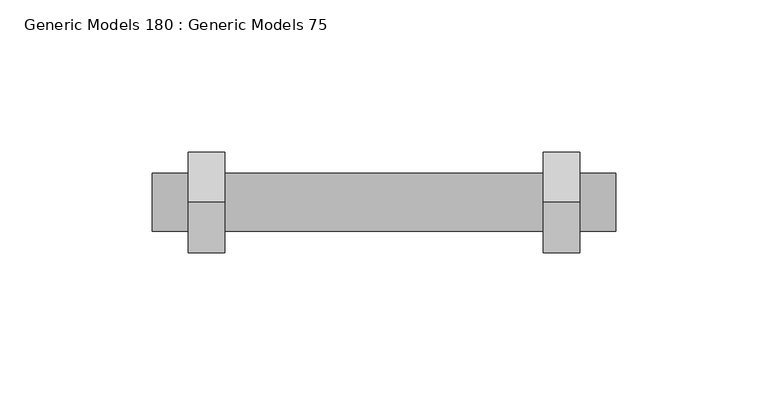
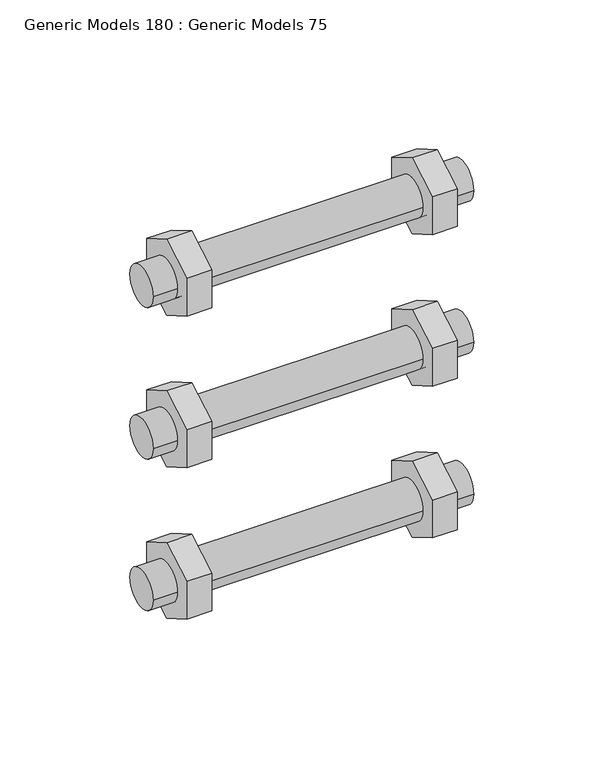
"""IFC4 building model written with IfcOpenShell, lengths in millimetres: proxy geometry, Generic Models 180 : Generic Models 75."""

from ifc_helpers import new_model, si_unit, point, frame, frame_2d, origin, place, context, project, spatial, polyline, circle_curve, trimmed, segment, composite_curve, outline, extrude, source, transform, mapped, element, save


def generic_models_180_generic_models_75_568aabff(model_context):
    return source(origin(), model_context, "Body", "SweptSolid", [
        extrude(outline(polyline([(30912.6241273, 269062.859622), (30929.1219112, 269072.384622), (30945.6196951, 269062.859622), (30945.6196951, 269043.809622), (30929.1219112, 269034.284622), (30912.6241273, 269043.809622), (30912.6241273, 269062.859622)])), frame((31918.2596032, 0.0, 0.0), z_axis=(1.0, 0.0, 0.0), x_axis=(0.0, 1.0, 0.0)), (0.0, 0.0, 1.0), 11.90625),
        extrude(outline(polyline([(30912.6241273, 268986.659622), (30929.1219112, 268996.184622), (30945.6196951, 268986.659622), (30945.6196951, 268967.609622), (30929.1219112, 268958.084622), (30912.6241273, 268967.609622), (30912.6241273, 268986.659622)])), frame((31918.2596032, 0.0, 0.0), z_axis=(1.0, 0.0, 0.0), x_axis=(0.0, 1.0, 0.0)), (0.0, 0.0, 1.0), 11.90625),
        extrude(outline(polyline([(30912.6241273, 268910.459622), (30929.1219112, 268919.984622), (30945.6196951, 268910.459622), (30945.6196951, 268891.409622), (30929.1219112, 268881.884622), (30912.6241273, 268891.409622), (30912.6241273, 268910.459622)])), frame((31918.2596032, 0.0, 0.0), z_axis=(1.0, 0.0, 0.0), x_axis=(0.0, 1.0, 0.0)), (0.0, 0.0, 1.0), 11.90625),
        extrude(outline(polyline([(30912.6241273, 269062.859622), (30929.1219112, 269072.384622), (30945.6196951, 269062.859622), (30945.6196951, 269043.809622), (30929.1219112, 269034.284622), (30912.6241273, 269043.809622), (30912.6241273, 269062.859622)])), frame((31801.5783532, 0.0, 0.0), z_axis=(1.0, 0.0, 0.0), x_axis=(0.0, 1.0, 0.0)), (0.0, 0.0, 1.0), 11.90625),
        extrude(outline(polyline([(30912.6241273, 268986.659622), (30929.1219112, 268996.184622), (30945.6196951, 268986.659622), (30945.6196951, 268967.609622), (30929.1219112, 268958.084622), (30912.6241273, 268967.609622), (30912.6241273, 268986.659622)])), frame((31801.5783532, 0.0, 0.0), z_axis=(1.0, 0.0, 0.0), x_axis=(0.0, 1.0, 0.0)), (0.0, 0.0, 1.0), 11.90625),
        extrude(outline(polyline([(30912.6241273, 268910.459622), (30929.1219112, 268919.984622), (30945.6196951, 268910.459622), (30945.6196951, 268891.409622), (30929.1219112, 268881.884622), (30912.6241273, 268891.409622), (30912.6241273, 268910.459622)])), frame((31801.5783532, 0.0, 0.0), z_axis=(1.0, 0.0, 0.0), x_axis=(0.0, 1.0, 0.0)), (0.0, 0.0, 1.0), 11.90625),
        extrude(outline(composite_curve([segment(trimmed(circle_curve(frame_2d((30929.1219112, 268977.134622)), 9.525), [point((30938.6469112, 268977.134622))], [point((30919.5969112, 268977.134622))], False, "CARTESIAN"), True, "CONTINUOUS"), segment(trimmed(circle_curve(frame_2d((30929.1219112, 268977.134622)), 9.525), [point((30919.5969112, 268977.134622))], [point((30938.6469112, 268977.134622))], False, "CARTESIAN"), True, "CONTINUOUS")], self_intersect=False)), frame((31789.6721032, 0.0, 0.0), z_axis=(1.0, 0.0, 0.0), x_axis=(0.0, 1.0, 0.0)), (0.0, 0.0, 1.0), 152.4),
        extrude(outline(composite_curve([segment(trimmed(circle_curve(frame_2d((30929.1219112, 268900.934622)), 9.525), [point((30938.6469112, 268900.934622))], [point((30919.5969112, 268900.934622))], False, "CARTESIAN"), True, "CONTINUOUS"), segment(trimmed(circle_curve(frame_2d((30929.1219112, 268900.934622)), 9.525), [point((30919.5969112, 268900.934622))], [point((30938.6469112, 268900.934622))], False, "CARTESIAN"), True, "CONTINUOUS")], self_intersect=False)), frame((31789.6721032, 0.0, 0.0), z_axis=(1.0, 0.0, 0.0), x_axis=(0.0, 1.0, 0.0)), (0.0, 0.0, 1.0), 152.4),
        extrude(outline(composite_curve([segment(trimmed(circle_curve(frame_2d((30929.1219112, 269053.334622)), 9.525), [point((30938.6469112, 269053.334622))], [point((30919.5969112, 269053.334622))], False, "CARTESIAN"), True, "CONTINUOUS"), segment(trimmed(circle_curve(frame_2d((30929.1219112, 269053.334622)), 9.525), [point((30919.5969112, 269053.334622))], [point((30938.6469112, 269053.334622))], False, "CARTESIAN"), True, "CONTINUOUS")], self_intersect=False)), frame((31789.6721032, 0.0, 0.0), z_axis=(1.0, 0.0, 0.0), x_axis=(0.0, 1.0, 0.0)), (0.0, 0.0, 1.0), 152.4),
    ])


if __name__ == "__main__":
    model = new_model("IFC4")
    model_context = context("Model", 3, world=origin())
    ifc_project = project(units=[si_unit("LENGTHUNIT", "METRE", prefix="MILLI")], contexts=[model_context])
    site = spatial("IfcSite", under=ifc_project)
    building = spatial("IfcBuilding", under=site)
    placement = place(None, origin())
    generic_models_180_generic_models_75_shape = generic_models_180_generic_models_75_568aabff(model_context)
    element("IfcBuildingElementProxy", 1, Name="Generic Models 180 : Generic Models 75", ObjectType="Generic Models 180 : Generic Models 75", at=placement, inside=building, context=model_context, shape_type="MappedRepresentation", body=[
        mapped(generic_models_180_generic_models_75_shape, transform((0.0, 0.0, 0.0), x_axis=(1.0, 0.0, 0.0), y_axis=(0.0, 1.0, 0.0), z_axis=(0.0, 0.0, 1.0))),
    ])
    save(model, "model.ifc")
